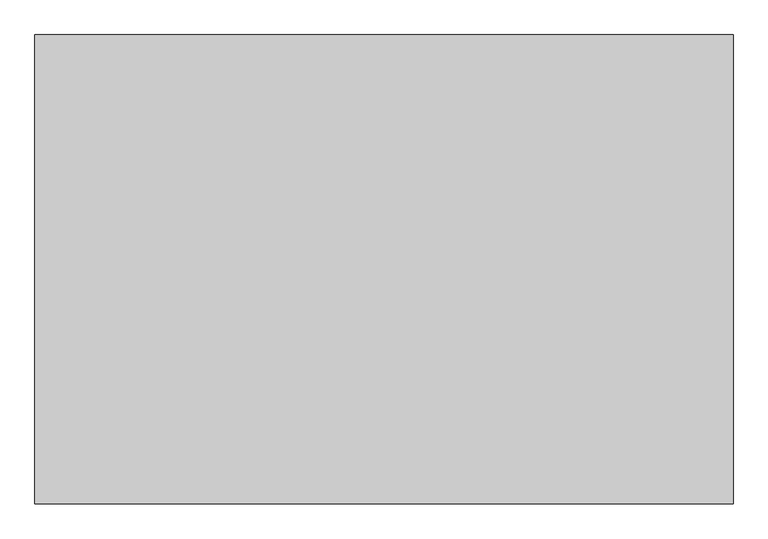
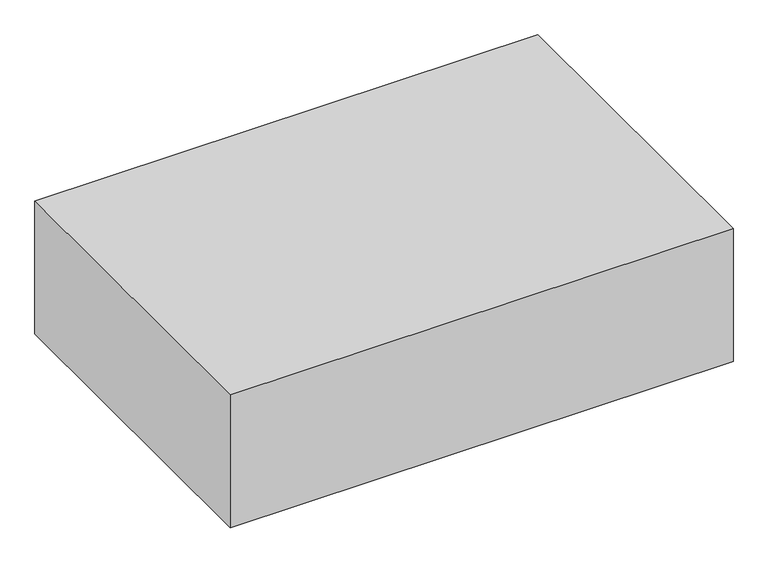
"""IFC4 building model written with IfcOpenShell, lengths in millimetres: proxy geometry, Space Planning Box_hec : Space Planning Box_hec."""

from ifc_helpers import new_model, si_unit, origin, origin_with_axes, place, context, project, spatial, polyline, outline, extrude, source, transform, mapped, element, save


def generic_models_608d95d2(model_context):
    return source(origin(), model_context, "Body", "SweptSolid", [
        extrude(outline(polyline([(9300.0, 6250.0), (9300.0, -6250.0), (-9300.0, -6250.0), (-9300.0, 6250.0), (9300.0, 6250.0)])), origin_with_axes(), (0.0, 0.0, 1.0), 5200.0),
    ])


if __name__ == "__main__":
    model = new_model("IFC4")
    model_context = context("Model", 3, world=origin())
    ifc_project = project(units=[si_unit("LENGTHUNIT", "METRE", prefix="MILLI")], contexts=[model_context])
    site = spatial("IfcSite", under=ifc_project)
    building = spatial("IfcBuilding", under=site)
    placement = place(None, origin())
    generic_models_shape = generic_models_608d95d2(model_context)
    element("IfcBuildingElementProxy", 1, Name="Space Planning Box_hec : Space Planning Box_hec", ObjectType="Space Planning Box_hec : Space Planning Box_hec", at=placement, inside=building, context=model_context, shape_type="MappedRepresentation", body=[
        mapped(generic_models_shape, transform((0.0, 0.0, 0.0), x_axis=(1.0, 0.0, 0.0), y_axis=(0.0, 1.0, 0.0), z_axis=(0.0, 0.0, 1.0))),
    ])
    save(model, "model.ifc")

# Revit data of these elements
# Type "Space Planning Box_hec : Space Planning Box_hec"
#   Type Comments = "..."
#   Room Name [instance default] = "?"
#   Interior Finish [instance default] = ""
#   Exterior Finish [instance default] = ""
#   Department [instance default] = ""
#   Assembly Code = "..."
#   ceiling height [instance default] = 0
#   Width [instance default] = 1524 mm
#   Program Area [instance default] = 0.00 m²
#   Length [instance default] = 1524 mm
#   Height [instance default] = 1524 mm
#   Area [instance default] = 2.32258 m²
#   Fill Color [instance default] = Cyan
#   Default Elevation = 0
# Element 1 (IfcBuildingElementProxy, "Space Planning Box_hec : Space Planning Box_hec")
#   Room Name = "HVAC Room"
#   Interior Finish = "IW1..N/A,,WB1..N/A,,FL2..N/A,,CL1..N/A"
#   Exterior Finish = "RF1..N/A,,EW1..N/A"
#   Department = "HV"
#   Width = 18600 mm
#   Program Area = 232.50 m²
#   Length = 12500 mm
#   Height = 5200 mm
#   Area = 232.50 m²
#   Fill Color = Lime
#   Materials on its faces: "Lime"
# Materials
#   "Cyan": class "Generic", colour RGB 0 255 255, transparency 0.2, Cost = 0
#   "Lime": class "Generic", colour RGB 0 255 0, transparency 0.2, Cost = 0
